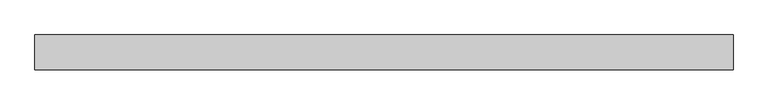
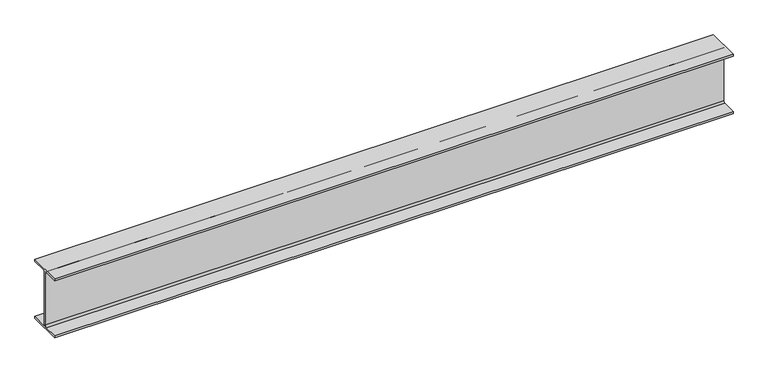
"""IFC4 building model written with IfcOpenShell, lengths in millimetres: beam geometry, Old_Steel Beam_H-KSD3502 : H_SB_ASB_H-200×200x8x12."""

from ifc_helpers import new_model, si_unit, point, frame, frame_2d, origin, place, context, project, spatial, polyline, circle_curve, trimmed, segment, composite_curve, outline, extrude, source, transform, mapped, element, save


def beam_561cba6f(model_context):
    return source(origin(), model_context, "Body", "SweptSolid", [
        extrude(outline(composite_curve([segment(polyline([(82.5, -141.5), (82.5, -151.7), (-82.5, -151.7), (-82.5, -141.5), (-11.9, -141.5)]), True, "CONTINUOUS"), segment(trimmed(circle_curve(frame_2d((-11.9, -132.6)), 8.9), [point((-11.9, -141.5))], [point((-3.0, -132.6))], True, "CARTESIAN"), True, "CONTINUOUS"), segment(polyline([(-3.0, -132.6), (-3.0, 132.6)]), True, "CONTINUOUS"), segment(trimmed(circle_curve(frame_2d((-11.9, 132.6)), 8.9), [point((-3.0, 132.6))], [point((-11.9, 141.5))], True, "CARTESIAN"), True, "CONTINUOUS"), segment(polyline([(-11.9, 141.5), (-82.5, 141.5), (-82.5, 151.7), (82.5, 151.7), (82.5, 141.5), (11.9, 141.5)]), True, "CONTINUOUS"), segment(trimmed(circle_curve(frame_2d((11.9, 132.6)), 8.9), [point((11.9, 141.5))], [point((3.0, 132.6))], True, "CARTESIAN"), True, "CONTINUOUS"), segment(polyline([(3.0, 132.6), (3.0, -132.6)]), True, "CONTINUOUS"), segment(trimmed(circle_curve(frame_2d((11.9, -132.6)), 8.9), [point((3.0, -132.6))], [point((11.9, -141.5))], True, "CARTESIAN"), True, "CONTINUOUS"), segment(polyline([(11.9, -141.5), (82.5, -141.5)]), True, "CONTINUOUS")], self_intersect=False)), frame((-1695.2828606, 0.0, 0.0), z_axis=(1.0, 0.0, 0.0), x_axis=(0.0, 1.0, 0.0)), (0.0, 0.0, 1.0), 3284.9531949),
    ])


if __name__ == "__main__":
    model = new_model("IFC4")
    model_context = context("Model", 3, world=origin())
    ifc_project = project(units=[si_unit("LENGTHUNIT", "METRE", prefix="MILLI")], contexts=[model_context])
    site = spatial("IfcSite", under=ifc_project)
    building = spatial("IfcBuilding", under=site)
    placement = place(None, origin())
    beam_shape = beam_561cba6f(model_context)
    element("IfcBeam", 1, ObjectType="Old_Steel Beam_H-KSD3502 : H_SB_ASB_H-200×200x8x12", at=placement, inside=building, context=model_context, shape_type="MappedRepresentation", body=[
        mapped(beam_shape, transform((0.0, 0.0, 0.0), x_axis=(1.0, 0.0, 0.0), y_axis=(0.0, 1.0, 0.0), z_axis=(0.0, 0.0, 1.0))),
    ])
    save(model, "model.ifc")

# Revit data of these elements
# Type "Old_Steel Beam_H-KSD3502 : H_SB_ASB_H-200×200x8x12"
#   Width = 20.0 cm
#   Web Thickness = 0.8 cm
#   Web Fillet = 1.3 cm
#   Warping Constant = 141376.0 cm⁶
#   Torsional Moment of Inertia = 26.2485 cm⁴
#   Torsional Modulus = 1.0 cm³
#   Section Area = 63.53 cm²
#   Plastic Modulus weak axis = 244.0 cm³
#   Plastic Modulus strong axis = 525.0 cm³
#   Perimeter = 1.16 m²/m
#   Nominal Weight = 49.90 kgf/m
#   Moment of Inertia weak axis = 1600.00 cm⁴
#   Moment of Inertia strong axis = 4720.00 cm⁴
#   Height = 20.0 cm
#   Flange Thickness = 1.2 cm
#   Elastic Modulus weak axis = 160.0 cm³
#   Elastic Modulus strong axis = 472.0 cm³
#   Centroid Vertical = 10.0 cm
#   Centroid Horizontal = 10.0 cm
#   Length [instance default] = 1.5240 m
#   Structural Material [instance default] = Steel, 45-345
#   Assembly Code = ""
# Element 1 (IfcBeam, "Old_Steel Beam_H-KSD3502 : H_SB_ASB_H-200×200x8x12")
#   Structural Material = none
# Materials
#   "Steel, 45-345": class "Metal", colour RGB 189 187 185, transparency 0, Description = "Steel 345 MPa", Cost = 0
